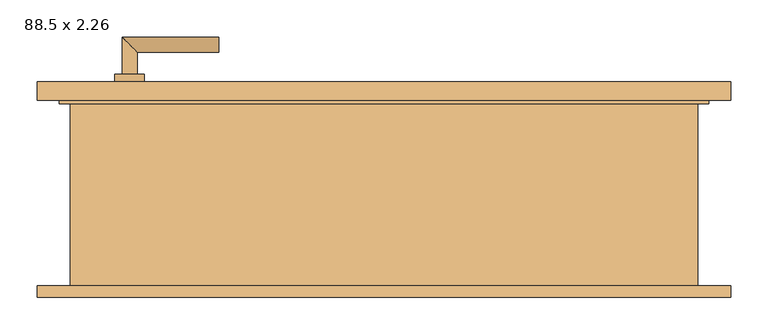
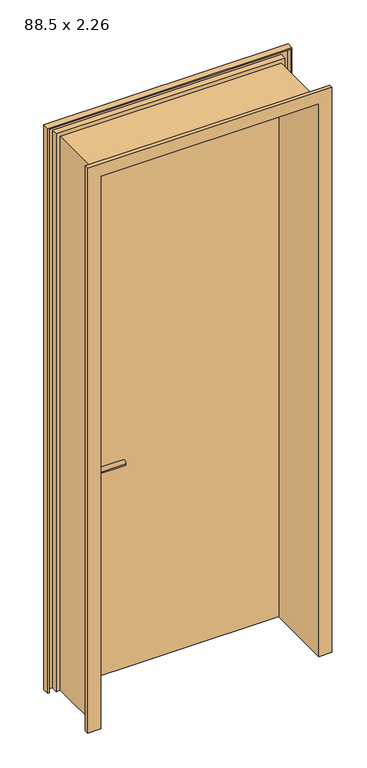
"""IFC4 building model written with IfcOpenShell, lengths in millimetres: door geometry, Drehflügel 1-flg - Stahlzarge : 88.5 x 2.26."""

import ifcopenshell
import ifcopenshell.guid

model = None  # the IFC model being written
_history = None  # IfcOwnerHistory: only IFC2X3 demands one
_inside = {}  # id of a spatial element -> (the spatial element, [elements in it])
_under = {}  # id of a project, library or spatial element -> (it, [spatial elements below it])
_declared = {}  # id of a project -> (the project, [libraries it declares])
_typed = {}  # id of a type object -> (the type object, [elements of that type])
_made_of = {}  # id of a material, layer set ... -> (it, [elements and type objects made of it])


def new_model(schema):
    """Start an empty IFC model of exactly this schema.

    Asked for "IFC4X3", IfcOpenShell would pick the latest addendum, in which some entities
    have other attributes; the version numbers below select the first issue.
    IFC2X3 requires an IfcOwnerHistory on every rooted entity: one is made here for all.
    """
    global model, _history
    if schema == "IFC4X3":
        model = ifcopenshell.file(schema_version=(4, 3, 0, 0))
    else:
        model = ifcopenshell.file(schema=schema)
    _inside.clear()
    _under.clear()
    _declared.clear()
    _typed.clear()
    _made_of.clear()
    _history = None
    if model.schema == "IFC2X3":
        org = make("IfcOrganization", Name="unknown")
        user = make(
            "IfcPersonAndOrganization",
            ThePerson=make("IfcPerson", FamilyName="unknown"),
            TheOrganization=org,
        )
        app = make(
            "IfcApplication",
            ApplicationDeveloper=org,
            Version="unknown",
            ApplicationFullName="unknown",
            ApplicationIdentifier="unknown",
        )
        _history = make(
            "IfcOwnerHistory",
            OwningUser=user,
            OwningApplication=app,
            ChangeAction="ADDED",
            CreationDate=0,
        )
    return model


def make(cls, **values):
    """One entity of the class cls with the attributes given. An attribute that is None is left unset."""
    return model.create_entity(
        cls, **{name: value for name, value in values.items() if value is not None}
    )


def rooted(cls, **values):
    """An entity with a GlobalId (a new one), such as an element, a storey or a relation."""
    return make(cls, GlobalId=ifcopenshell.guid.new(), OwnerHistory=_history, **values)


def si_unit(unit_type, name, prefix=None):
    """IfcSIUnit, for example si_unit("LENGTHUNIT", "METRE", prefix="MILLI")."""
    return make("IfcSIUnit", UnitType=unit_type, Prefix=prefix, Name=name)


def assignment(units):
    """IfcUnitAssignment: the units of a project."""
    return None if units is None else make("IfcUnitAssignment", Units=units)


def point(xyz):
    """IfcCartesianPoint."""
    return None if xyz is None else make("IfcCartesianPoint", Coordinates=xyz)


def direction(xyz):
    """IfcDirection."""
    return None if xyz is None else make("IfcDirection", DirectionRatios=xyz)


def frame(location, z_axis=None, x_axis=None):
    """IfcAxis2Placement3D, a coordinate frame: its origin and axes. An axis left out is left unset."""
    return make(
        "IfcAxis2Placement3D",
        Location=point(location),
        Axis=direction(z_axis),
        RefDirection=direction(x_axis),
    )


def frame_2d(location, x_axis=None):
    """IfcAxis2Placement2D, a coordinate frame in the plane: its origin and x axis."""
    return make(
        "IfcAxis2Placement2D", Location=point(location), RefDirection=direction(x_axis)
    )


def origin():
    """The frame at (0, 0, 0) with its axes left unset."""
    return frame((0.0, 0.0, 0.0))


def place(relative_to, where):
    """IfcLocalPlacement: puts the frame where relative to a parent placement (None: the world)."""
    return make(
        "IfcLocalPlacement", PlacementRelTo=relative_to, RelativePlacement=where
    )


def context(
    kind, dimensions, precision=None, world=None, true_north=None, identifier=None
):
    """IfcGeometricRepresentationContext, for example the 3D "Model" context."""
    return make(
        "IfcGeometricRepresentationContext",
        ContextIdentifier=identifier,
        ContextType=kind,
        CoordinateSpaceDimension=dimensions,
        Precision=precision,
        WorldCoordinateSystem=world,
        TrueNorth=true_north,
    )


def project(units=None, contexts=None):
    """IfcProject with its units and contexts."""
    return rooted(
        "IfcProject",
        Name="project",
        RepresentationContexts=contexts,
        UnitsInContext=assignment(units),
    )


def spatial(cls, under=None, at=None, **own):
    """A site, building, storey or space (cls), placed at a placement, below another one or the project."""
    s = rooted(cls, ObjectPlacement=at, **own)
    if under is not None:
        _under.setdefault(under.id(), (under, []))[1].append(s)
    return s


def polyline(points):
    """IfcPolyline through the points."""
    return make("IfcPolyline", Points=[point(p) for p in points])


def circle_curve(where, radius):
    """IfcCircle in the frame where."""
    return make("IfcCircle", Position=where, Radius=radius)


def ellipse_curve(where, semi_axis1, semi_axis2):
    """IfcEllipse in the frame where."""
    return make(
        "IfcEllipse", Position=where, SemiAxis1=semi_axis1, SemiAxis2=semi_axis2
    )


def trimmed(basis, trim1, trim2, sense, master):
    """IfcTrimmedCurve: the piece of a basis curve between two trims."""
    return make(
        "IfcTrimmedCurve",
        BasisCurve=basis,
        Trim1=trim1,
        Trim2=trim2,
        SenseAgreement=sense,
        MasterRepresentation=master,
    )


def segment(curve, same_sense, transition):
    """IfcCompositeCurveSegment."""
    return make(
        "IfcCompositeCurveSegment",
        Transition=transition,
        SameSense=same_sense,
        ParentCurve=curve,
    )


def composite_curve(segments, self_intersect=None):
    """IfcCompositeCurve: segments joined end to end."""
    return make("IfcCompositeCurve", Segments=segments, SelfIntersect=self_intersect)


def outline(outer, holes=None, kind="AREA"):
    """IfcArbitraryClosedProfileDef: a profile drawn as a closed curve; with holes, ...WithVoids."""
    if holes is None:
        return make("IfcArbitraryClosedProfileDef", ProfileType=kind, OuterCurve=outer)
    return make(
        "IfcArbitraryProfileDefWithVoids",
        ProfileType=kind,
        OuterCurve=outer,
        InnerCurves=holes,
    )


def extrude(swept, where, along, depth):
    """IfcExtrudedAreaSolid: the profile swept, set in the frame where, extruded along a direction by depth."""
    return make(
        "IfcExtrudedAreaSolid",
        SweptArea=swept,
        Position=where,
        ExtrudedDirection=direction(along),
        Depth=depth,
    )


def faces_of(points, faces, orient=None, outer=None):
    """IfcFace entities. A face is a list of loops; a loop is a list of indices into points, from 0.

    orient and outer hold one flag for each loop. By default every Orientation is true, the
    first loop of a face is its IfcFaceOuterBound and the others are IfcFaceBound.
    """
    made = []
    for i, loops in enumerate(faces):
        bounds = []
        for j, loop in enumerate(loops):
            is_outer = j == 0 if outer is None else outer[i][j]
            bounds.append(
                make(
                    "IfcFaceOuterBound" if is_outer else "IfcFaceBound",
                    Bound=make("IfcPolyLoop", Polygon=[points[k] for k in loop]),
                    Orientation=True if orient is None else orient[i][j],
                )
            )
        made.append(make("IfcFace", Bounds=bounds))
    return made


def faceted_brep(points, faces, orient=None, outer=None, voids=None):
    """IfcFacetedBrep: a solid bounded by flat faces; with voids (closed shells), ...WithVoids."""
    shared = [point(p) for p in points]
    hull = make("IfcClosedShell", CfsFaces=faces_of(shared, faces, orient, outer))
    if voids is None:
        return make("IfcFacetedBrep", Outer=hull)
    return make(
        "IfcFacetedBrepWithVoids",
        Outer=hull,
        Voids=[
            make(cls, CfsFaces=faces_of(shared, fs, o, b)) for cls, fs, o, b in voids
        ],
    )


def shape(context_of_items, identifier, shape_type, items):
    """IfcShapeRepresentation: the items that make up one representation, for example the "Body"."""
    return make(
        "IfcShapeRepresentation",
        ContextOfItems=context_of_items,
        RepresentationIdentifier=identifier,
        RepresentationType=shape_type,
        Items=items,
    )


def source(mapping_origin, context_of_items, identifier, shape_type, items):
    """IfcRepresentationMap: a shape defined once, which mapped items show again and again."""
    return make(
        "IfcRepresentationMap",
        MappingOrigin=mapping_origin,
        MappedRepresentation=shape(context_of_items, identifier, shape_type, items),
    )


def transform(
    local_origin,
    x_axis=None,
    y_axis=None,
    z_axis=None,
    scale=None,
    scale2=None,
    scale3=None,
    uniform=True,
):
    """IfcCartesianTransformationOperator3D, or its non-uniform kind. x_axis, y_axis, z_axis: its Axis1, 2, 3."""
    if uniform:
        return make(
            "IfcCartesianTransformationOperator3D",
            Axis1=direction(x_axis),
            Axis2=direction(y_axis),
            LocalOrigin=point(local_origin),
            Scale=scale,
            Axis3=direction(z_axis),
        )
    return make(
        "IfcCartesianTransformationOperator3DnonUniform",
        Axis1=direction(x_axis),
        Axis2=direction(y_axis),
        LocalOrigin=point(local_origin),
        Scale=scale,
        Axis3=direction(z_axis),
        Scale2=scale2,
        Scale3=scale3,
    )


def mapped(mapping_source, mapping_target):
    """IfcMappedItem: shows the shape of a source again, moved by a transform."""
    return make(
        "IfcMappedItem", MappingSource=mapping_source, MappingTarget=mapping_target
    )


def made_of(thing, what):
    """Note that an element or type object is made of a material, layer set ...; save() writes the relation."""
    if what is not None:
        _made_of.setdefault(what.id(), (what, []))[1].append(thing)
    return thing


def element(
    cls,
    number,
    at=None,
    inside=None,
    cuts=None,
    type_object=None,
    material=None,
    context=None,
    identifier="Body",
    shape_type=None,
    held_by="IfcProductDefinitionShape",
    body=None,
    shapes=None,
    **own,
):
    """One element of the class cls, such as IfcWall. Its Tag is "e" and its number.

    at: its placement. inside: the storey or other place that contains it. cuts: it is an
    opening in that element (IfcRelVoidsElement). A single representation is given by context,
    identifier, shape_type and body (its items); several are given by shapes. held_by: the class
    of the entity that holds the representations. save() writes the other relations.
    """
    e = rooted(cls, Tag="e%d" % number, ObjectPlacement=at, **own)
    if body is not None:
        shapes = [shape(context, identifier, shape_type, body)]
    if shapes is not None:
        e.Representation = make(held_by, Representations=shapes)
    if inside is not None:
        _inside.setdefault(inside.id(), (inside, []))[1].append(e)
    if cuts is not None:
        rooted(
            "IfcRelVoidsElement", RelatingBuildingElement=cuts, RelatedOpeningElement=e
        )
    if type_object is not None:
        _typed.setdefault(type_object.id(), (type_object, []))[1].append(e)
    return made_of(e, material)


def aggregate(whole, parts):
    """IfcRelAggregates: a whole, such as a stair, and the parts it consists of."""
    return rooted("IfcRelAggregates", RelatingObject=whole, RelatedObjects=parts)


def save(model, path):
    """Write the relations noted so far, then the file.

    IfcRelAggregates (storeys below a building ...), IfcRelContainedInSpatialStructure (elements
    in a storey), IfcRelDefinesByType, IfcRelAssociatesMaterial and IfcRelDeclares: one each for
    every whole, place, type object, material and project.
    """
    for whole, parts in _under.values():
        aggregate(whole, parts)
    for where, things in _inside.values():
        rooted(
            "IfcRelContainedInSpatialStructure",
            RelatedElements=things,
            RelatingStructure=where,
        )
    for kind, things in _typed.values():
        rooted("IfcRelDefinesByType", RelatedObjects=things, RelatingType=kind)
    for what, things in _made_of.values():
        rooted("IfcRelAssociatesMaterial", RelatedObjects=things, RelatingMaterial=what)
    for by, libraries in _declared.values():
        rooted("IfcRelDeclares", RelatingContext=by, RelatedDefinitions=libraries)
    model.write(path)


def plane_surface(at):
    """IfcPlane: the flat surface through the origin of the frame at, square to its z axis."""
    return make("IfcPlane", Position=at)


def cylinder_surface(at, radius):
    """IfcCylindricalSurface: all points at the distance radius from the z axis of the frame at."""
    return make("IfcCylindricalSurface", Position=at, Radius=radius)


def advanced_brep(points, edges, surfaces, faces):
    """IfcAdvancedBrep: a solid bounded by faces that lie on surfaces and meet in shared edges.

    An edge is (start, end): straight between two places in points (the first is 0);
    or (start, end, curve); or (start, end, curve, False) where it runs against its curve.
    A face is (place in surfaces, loops), or (place, loops, False) where it looks against
    its surface's normal. A loop lists edges by number (the first is 1), with a minus sign
    where the edge is run from its end to its start. The first loop is the outer one.
    """
    corners = [point(p) for p in points]
    vertices = [make("IfcVertexPoint", VertexGeometry=c) for c in corners]
    made = []
    for start, end, *more in edges:
        made.append(
            make(
                "IfcEdgeCurve",
                EdgeStart=vertices[start],
                EdgeEnd=vertices[end],
                EdgeGeometry=more[0] if more else make("IfcPolyline", Points=[corners[start], corners[end]]),
                SameSense=more[1] if len(more) > 1 else True,
            )
        )
    hull = []
    for where, loops, *sense in faces:
        bounds = []
        for j, loop in enumerate(loops):
            ring = [make("IfcOrientedEdge", EdgeElement=made[abs(k) - 1], Orientation=k > 0) for k in loop]
            bounds.append(
                make(
                    "IfcFaceOuterBound" if j == 0 else "IfcFaceBound",
                    Bound=make("IfcEdgeLoop", EdgeList=ring),
                    Orientation=True,
                )
            )
        hull.append(make("IfcAdvancedFace", Bounds=bounds, FaceSurface=surfaces[where], SameSense=sense[0] if sense else True))
    return make("IfcAdvancedBrep", Outer=make("IfcClosedShell", CfsFaces=hull))


def door_88_5_x_2_26_01f20a05(model_context):
    return source(origin(), model_context, "Body", "SolidModel", [
        advanced_brep(
        [(-352.5, 114.4346141, 1000.0), (-332.5, 114.4346141, 1000.0), (-352.5, 44.4346141, 1000.0), (-332.5, 64.4346141, 1000.0), (-222.5, 44.4346141, 1000.0), (-222.5, 64.4346141, 1000.0)],
        [
            (0, 1, circle_curve(frame((-342.5, 114.4346141, 1000.0), z_axis=(0.0, 1.0, 0.0), x_axis=(1.0, 0.0, 0.0)), 10.0)),
            (1, 0, circle_curve(frame((-342.5, 114.4346141, 1000.0), z_axis=(0.0, 1.0, 0.0), x_axis=(1.0, 0.0, 0.0)), 10.0)),
            (0, 2),
            (2, 3, ellipse_curve(frame((-342.5, 54.4346141, 1000.0), z_axis=(-0.7071067811865385, 0.7071067811865565, 0.0), x_axis=(0.7071067811865563, 0.7071067811865386, 0.0)), 14.1421356, 10.0)),
            (3, 1),
            (3, 2, ellipse_curve(frame((-342.5, 54.4346141, 1000.0), z_axis=(-0.7071067811865385, 0.7071067811865565, 0.0), x_axis=(0.7071067811865563, 0.7071067811865386, 0.0)), 14.1421356, 10.0)),
            (4, 5, circle_curve(frame((-222.5, 54.4346141, 1000.0), z_axis=(1.0, 0.0, 0.0), x_axis=(0.0, 1.0, 0.0)), 10.0)),
            (5, 4, circle_curve(frame((-222.5, 54.4346141, 1000.0), z_axis=(1.0, 0.0, 0.0), x_axis=(0.0, 1.0, 0.0)), 10.0)),
            (2, 4),
            (5, 3),
        ],
        [
            plane_surface(frame((-342.5, 114.4346141, -287.7526403), z_axis=(0.0, 1.0, 0.0), x_axis=(0.0, 0.0, 1.0))),
            cylinder_surface(frame((-342.5, 114.4346141, 1000.0), z_axis=(0.0, 1.0, 0.0), x_axis=(1.0, 0.0, 0.0)), 10.0),
            plane_surface(frame((-222.5, 54.4346141, -287.7526403), z_axis=(1.0, 0.0, 0.0), x_axis=(0.0, 0.0, 1.0))),
            cylinder_surface(frame((-342.5, 54.4346141, 1000.0), z_axis=(-1.0, 0.0, 0.0), x_axis=(0.0, 1.0, 0.0)), 10.0),
        ],
        [
            (0, [[1, 2]]),
            (1, [[-1, 3, 4, 5]]),
            (1, [[-2, -5, 6, -3]]),
            (2, [[7, 8]]),
            (3, [[-4, 9, -8, 10]]),
            (3, [[-6, -10, -7, -9]]),
        ],
    ),
        advanced_brep(
        [(-332.5, 174.4346141, 1000.0), (-352.5, 174.4346141, 1000.0), (-332.5, 204.4346141, 1000.0), (-352.5, 224.4346141, 1000.0), (-222.5, 204.4346141, 1000.0), (-222.5, 224.4346141, 1000.0)],
        [
            (0, 1, circle_curve(frame((-342.5, 174.4346141, 1000.0), z_axis=(0.0, -1.0, 0.0), x_axis=(-1.0, 0.0, 0.0)), 10.0)),
            (1, 0, circle_curve(frame((-342.5, 174.4346141, 1000.0), z_axis=(0.0, -1.0, 0.0), x_axis=(-1.0, 0.0, 0.0)), 10.0)),
            (0, 2),
            (2, 3, ellipse_curve(frame((-342.5, 214.4346141, 1000.0), z_axis=(-0.7071067811865475, -0.7071067811865475, 0.0), x_axis=(0.7071067811865474, -0.7071067811865476, 0.0)), 14.1421356, 10.0)),
            (3, 1),
            (3, 2, ellipse_curve(frame((-342.5, 214.4346141, 1000.0), z_axis=(-0.7071067811865475, -0.7071067811865475, 0.0), x_axis=(0.7071067811865474, -0.7071067811865476, 0.0)), 14.1421356, 10.0)),
            (4, 5, circle_curve(frame((-222.5, 214.4346141, 1000.0), z_axis=(1.0, 0.0, 0.0), x_axis=(0.0, 1.0, 0.0)), 10.0)),
            (5, 4, circle_curve(frame((-222.5, 214.4346141, 1000.0), z_axis=(1.0, 0.0, 0.0), x_axis=(0.0, 1.0, 0.0)), 10.0)),
            (2, 4),
            (5, 3),
        ],
        [
            plane_surface(frame((-342.5, 174.4346141, -287.7526403), z_axis=(0.0, -1.0, 0.0), x_axis=(0.0, 0.0, 1.0))),
            cylinder_surface(frame((-342.5, 174.4346141, 1000.0), z_axis=(0.0, -1.0, 0.0), x_axis=(-1.0, 0.0, 0.0)), 10.0),
            plane_surface(frame((-222.5, 214.4346141, -287.7526403), z_axis=(1.0, 0.0, 0.0), x_axis=(0.0, 0.0, 1.0))),
            cylinder_surface(frame((-342.5, 214.4346141, 1000.0), z_axis=(-1.0, 0.0, 0.0), x_axis=(0.0, 1.0, 0.0)), 10.0),
        ],
        [
            (0, [[1, 2]]),
            (1, [[-1, 3, 4, 5]]),
            (1, [[-2, -5, 6, -3]]),
            (2, [[7, 8]]),
            (3, [[-4, 9, -8, 10]]),
            (3, [[-6, -10, -7, -9]]),
        ],
    ),
        extrude(outline(composite_curve([segment(trimmed(circle_curve(frame_2d((1000.0, -342.5)), 20.0), [point((1000.0, -362.5))], [point((1000.0, -322.5))], False, "CARTESIAN"), True, "CONTINUOUS"), segment(trimmed(circle_curve(frame_2d((1000.0, -342.5)), 20.0), [point((1000.0, -322.5))], [point((1000.0, -362.5))], False, "CARTESIAN"), True, "CONTINUOUS")], self_intersect=False)), frame((0.0, 104.4346141, 0.0), z_axis=(0.0, 1.0, 0.0), x_axis=(0.0, 0.0, 1.0)), (0.0, 0.0, 1.0), 10.0),
        extrude(outline(composite_curve([segment(trimmed(circle_curve(frame_2d((1000.0, -342.5)), 20.0), [point((1000.0, -362.5))], [point((1000.0, -322.5))], False, "CARTESIAN"), True, "CONTINUOUS"), segment(trimmed(circle_curve(frame_2d((1000.0, -342.5)), 20.0), [point((1000.0, -322.5))], [point((1000.0, -362.5))], False, "CARTESIAN"), True, "CONTINUOUS")], self_intersect=False)), frame((0.0, 164.4346141, 0.0), z_axis=(0.0, 1.0, 0.0), x_axis=(0.0, 0.0, 1.0)), (0.0, 0.0, 1.0), 10.0),
        extrude(outline(polyline([(432.5, 139.4346141), (-432.5, 139.4346141), (-432.5, 164.4346141), (432.5, 164.4346141), (432.5, 139.4346141)])), frame((0.0, 0.0, 100.0), z_axis=(0.0, 0.0, 1.0), x_axis=(1.0, 0.0, 0.0)), (0.0, 0.0, 1.0), 2250.0),
        faceted_brep([(466.9603207, -125.5653859, 100.0), (417.5, -125.5653859, 100.0), (417.5, 139.4346141, 100.0), (432.5, 139.4346141, 100.0), (432.5, 164.4346141, 100.0), (466.9603207, 164.4346141, 100.0), (466.9603207, 139.4346141, 100.0), (461.9603207, 139.4346141, 100.0), (461.9603207, 159.4346141, 100.0), (437.5, 159.4346141, 100.0), (437.5, 134.4346141, 100.0), (422.5, 134.4346141, 100.0), (422.5, -120.5653859, 100.0), (461.9603207, -120.5653859, 100.0), (461.9603207, -110.5653859, 100.0), (466.9603207, -110.5653859, 100.0), (466.9603207, -125.5653859, 2384.4603207), (-466.9603207, -125.5653859, 2384.4603207), (-466.9603207, -125.5653859, 100.0), (-417.5, -125.5653859, 100.0), (-417.5, -125.5653859, 2335.0), (417.5, -125.5653859, 2335.0), (417.5, 139.4346141, 2335.0), (-417.5, 139.4346141, 2335.0), (-417.5, 139.4346141, 100.0), (-432.5, 139.4346141, 100.0), (-432.5, 139.4346141, 2350.0), (432.5, 139.4346141, 2350.0), (432.5, 164.4346141, 2350.0), (-432.5, 164.4346141, 2350.0), (-432.5, 164.4346141, 100.0), (-466.9603207, 164.4346141, 100.0), (-466.9603207, 164.4346141, 2384.4603207), (466.9603207, 164.4346141, 2384.4603207), (466.9603207, 139.4346141, 2384.4603207), (-466.9603207, 139.4346141, 2384.4603207), (-466.9603207, 139.4346141, 100.0), (-461.9603207, 139.4346141, 100.0), (-461.9603207, 139.4346141, 2379.4603207), (461.9603207, 139.4346141, 2379.4603207), (461.9603207, 159.4346141, 2379.4603207), (-461.9603207, 159.4346141, 2379.4603207), (-461.9603207, 159.4346141, 100.0), (-437.5, 159.4346141, 100.0), (-437.5, 159.4346141, 2355.0), (437.5, 159.4346141, 2355.0), (437.5, 134.4346141, 2355.0), (-437.5, 134.4346141, 2355.0), (-437.5, 134.4346141, 100.0), (-422.5, 134.4346141, 100.0), (-422.5, 134.4346141, 2340.0), (422.5, 134.4346141, 2340.0), (422.5, -120.5653859, 2340.0), (-422.5, -120.5653859, 2340.0), (-422.5, -120.5653859, 100.0), (-461.9603207, -120.5653859, 100.0), (-461.9603207, -120.5653859, 2379.4603207), (461.9603207, -120.5653859, 2379.4603207), (461.9603207, -110.5653859, 2379.4603207), (-461.9603207, -110.5653859, 2379.4603207), (-461.9603207, -110.5653859, 100.0), (-466.9603207, -110.5653859, 100.0), (-466.9603207, -110.5653859, 2384.4603207), (466.9603207, -110.5653859, 2384.4603207)], [[[0, 1, 2, 3, 4, 5, 6, 7, 8, 9, 10, 11, 12, 13, 14, 15]], [[1, 0, 16, 17, 18, 19, 20, 21]], [[2, 1, 21, 22]], [[3, 2, 22, 23, 24, 25, 26, 27]], [[4, 3, 27, 28]], [[5, 4, 28, 29, 30, 31, 32, 33]], [[6, 5, 33, 34]], [[7, 6, 34, 35, 36, 37, 38, 39]], [[8, 7, 39, 40]], [[9, 8, 40, 41, 42, 43, 44, 45]], [[10, 9, 45, 46]], [[11, 10, 46, 47, 48, 49, 50, 51]], [[12, 11, 51, 52]], [[13, 12, 52, 53, 54, 55, 56, 57]], [[14, 13, 57, 58]], [[15, 14, 58, 59, 60, 61, 62, 63]], [[0, 15, 63, 16]], [[17, 62, 61, 18]], [[18, 61, 60, 55, 54, 49, 48, 43, 42, 37, 36, 31, 30, 25, 24, 19]], [[23, 20, 19, 24]], [[29, 26, 25, 30]], [[35, 32, 31, 36]], [[41, 38, 37, 42]], [[47, 44, 43, 48]], [[53, 50, 49, 54]], [[59, 56, 55, 60]], [[22, 21, 20, 23]], [[28, 27, 26, 29]], [[34, 33, 32, 35]], [[40, 39, 38, 41]], [[46, 45, 44, 47]], [[52, 51, 50, 53]], [[58, 57, 56, 59]], [[16, 63, 62, 17]]]),
    ])


if __name__ == "__main__":
    model = new_model("IFC4")
    model_context = context("Model", 3, world=origin())
    ifc_project = project(units=[si_unit("LENGTHUNIT", "METRE", prefix="MILLI")], contexts=[model_context])
    site = spatial("IfcSite", under=ifc_project)
    building = spatial("IfcBuilding", under=site)
    placement = place(None, origin())
    door_88_5_x_2_26_shape = door_88_5_x_2_26_01f20a05(model_context)
    element("IfcDoor", 1, ObjectType="Drehflügel 1-flg - Stahlzarge : 88.5 x 2.26", at=placement, inside=building, context=model_context, shape_type="MappedRepresentation", body=[
        mapped(door_88_5_x_2_26_shape, transform((0.0, 0.0, 0.0), x_axis=(1.0, 0.0, 0.0), y_axis=(0.0, 1.0, 0.0), z_axis=(0.0, 0.0, 1.0))),
    ])
    save(model, "model.ifc")

# Revit data of these elements
# Project information
#   Projektausgabedatum = "Projekt Datum"
#   Projektstatus = "Projektstatus"
#   Kundenname = "Bauherr"
#   Projektadresse = "Projektadresse"
#   Projektname = "Projektname"
#   Projektnummer = "Projektnummer"
#   Verfasser Firma 1 = "Firma 1"
#   Verfasser Firma 2 = "Firma 2"
#   Verfasser PLZ Ort = "PLZ Ort"
#   Verfasser Strasse = "Strasse"
#   Verfasser Telefon = "Telefon"
#   Verfasser Telefax = "Telefax"
#   Verfasser eMail = "E-Mail"
# Type "Drehflügel 1-flg - Stahlzarge : 88.5 x 2.26"
#   Type Mark = "21"
#   Operation = "SingleSwingRight"
#   Keynote = "16.03"
#   Analytic Construction = "Metall"
#   Thermal Resistance (R) = 0.270117 (m²·K)/W
#   Heat Transfer Coefficient (U) = 3.7021 W/(m²·K)
#   Rough Width = 0.885 m
#   Rough Height [instance default] = 2.360 m
#   Höhe Türgriff [instance default] = 0.900 m
#   Height = 2.260 m
#   Fußbodenaufbau [instance default] = 0.100 m
#   Width = 0.885 m
#   Sichtbarkeit Sturzlinien [instance default] = yes
#   Türgriff auswählen [instance default] = element 221079
#   Türgriff [instance default] = none
#   Türflügel [instance default] = none
#   Rahmen/Pfosten [instance default] = Metall - Lackiert - Grau
#   Visual Light Transmittance = 0
#   Solar Heat Gain Coefficient = 0
#   Function = (empty or 0)
#   Wall Closure = (empty or 0)
# Element 1 (IfcDoor, "Drehflügel 1-flg - Stahlzarge : 88.5 x 2.26")
#   Materials on its faces: "Metall - Lackiert - Grau", "Metall - Chrom", "Holz - Birke"
# Materials
#   "Metall - Lackiert - Grau": class "Farbe 1", colour RGB 98 98 98, transparency 0, Cost = 0
#   "Metall - Chrom": class "Metall", colour RGB 247 247 247, transparency 0, Cost = 0
#   "Holz - Birke": class "Holz", colour RGB 213 164 103, transparency 0, Cost = 0
